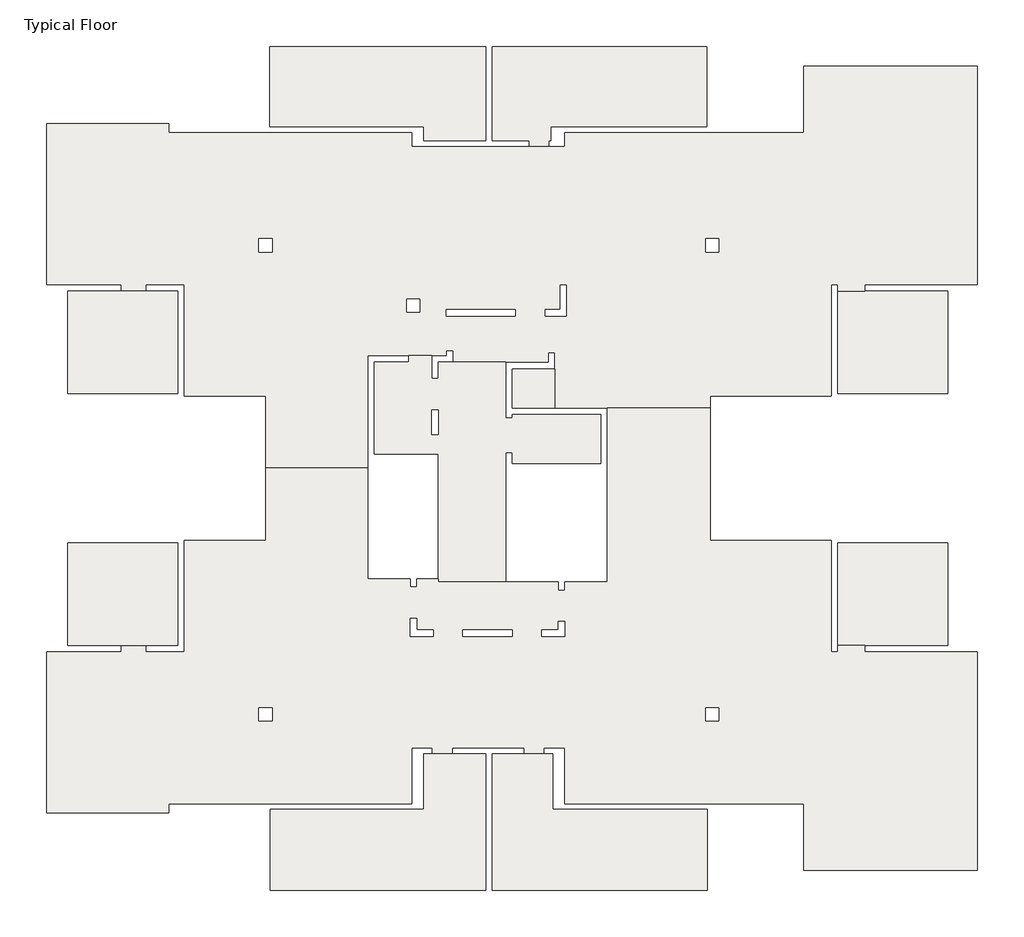
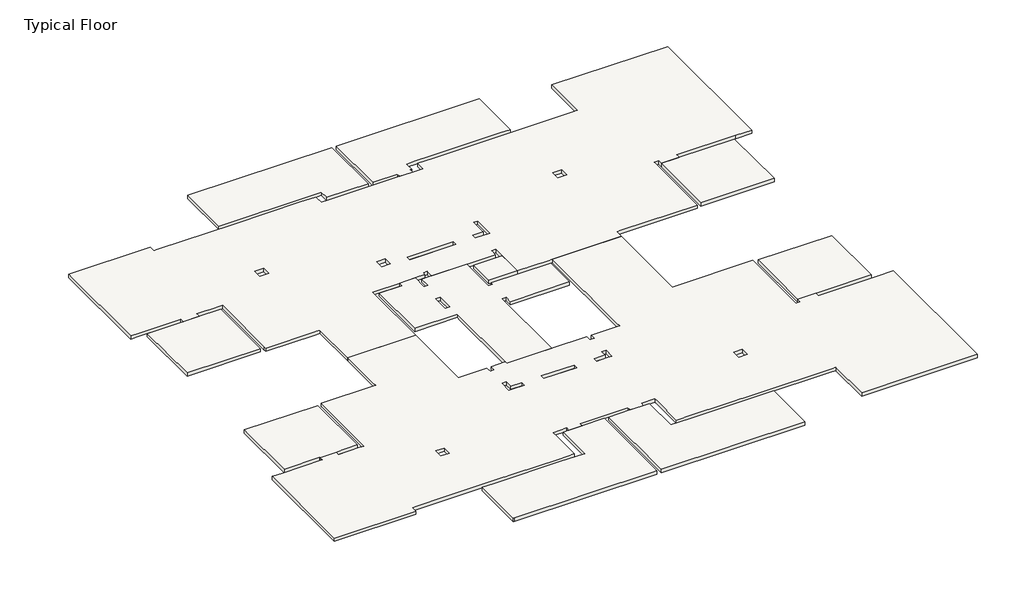
# One storey: 12 slabs.
"""IFC4 building model written with IfcOpenShell, lengths in millimetres."""

from ifc_helpers import new_model, si_unit, frame, origin, place, context, project, spatial, polyline, outline, extrude, faceted_brep, element, save

model = new_model("IFC4")

# Units and contexts
model_context = context("Model", 3, world=origin())
ifc_project = project(units=[si_unit("LENGTHUNIT", "METRE", prefix="MILLI")], contexts=[model_context])

# Site, building, storey
site = spatial("IfcSite", under=ifc_project)
building = spatial("IfcBuilding", under=site)
storey = spatial("IfcBuildingStorey", under=building, Name="Typical Floor", Elevation=3700.0)

# Slabs
placement = place(None, origin())
element("IfcSlab", 1, ObjectType="16", at=placement, inside=storey, context=model_context, shape_type="Brep", body=[
    faceted_brep([(-29879.8305532, 23917.9715458, 3540.0), (-29879.8305532, 26366.9840713, 3540.0), (-23307.4000343, 26366.9840713, 3540.0), (-23307.4000343, 23496.7461841, 3540.0), (-25199.7256887, 23496.7461841, 3540.0), (-25199.7256887, 23917.9715458, 3540.0), (-25559.7256887, 23917.9715458, 3540.0), (-26241.1471859, 23917.9715458, 3540.0), (-29280.7432632, 23917.9715458, 3540.0), (-29879.8305532, 26366.9840713, 3700.0), (-29879.8305532, 23917.9715458, 3700.0), (-29280.7432632, 23917.9715458, 3700.0), (-26241.1471859, 23917.9715458, 3700.0), (-25559.7256887, 23917.9715458, 3700.0), (-25199.7256887, 23917.9715458, 3700.0), (-25199.7256887, 23496.7461841, 3700.0), (-23307.4000343, 23496.7461841, 3700.0), (-23307.4000343, 26366.9840713, 3700.0)], [[[0, 1, 2, 3, 4, 5, 6, 7, 8]], [[9, 10, 11, 12, 13, 14, 15, 16, 17]], [[1, 0, 10, 9]], [[2, 1, 9, 17]], [[3, 2, 17, 16]], [[4, 3, 16, 15]], [[5, 4, 15, 14]], [[5, 14, 13, 12, 11, 10, 0, 8, 7, 6]]]),
])
element("IfcSlab", 2, ObjectType="16", at=placement, inside=storey, context=model_context, shape_type="Brep", body=[
    faceted_brep([(-21979.7256887, 23496.7461841, 3540.0), (-23107.4000343, 23496.7461841, 3540.0), (-23107.4000343, 26366.9840713, 3540.0), (-22980.4228437, 26366.9840713, 3540.0), (-16580.4228437, 26366.9840713, 3540.0), (-16580.4228437, 23917.8919264, 3540.0), (-17031.2403988, 23917.8919264, 3540.0), (-20181.0054246, 23917.8919264, 3540.0), (-20900.686947, 23917.8919264, 3540.0), (-21330.686947, 23917.8919264, 3540.0), (-21330.686947, 23496.7461841, 3540.0), (-21381.1801988, 23496.7461841, 3540.0), (-21381.1801988, 23316.6665647, 3540.0), (-21979.7256887, 23316.6665647, 3540.0), (-23107.4000343, 23496.7461841, 3700.0), (-21979.7256887, 23496.7461841, 3700.0), (-21979.7256887, 23316.6665647, 3700.0), (-21381.1801988, 23316.6665647, 3700.0), (-21381.1801988, 23496.7461841, 3700.0), (-21330.686947, 23496.7461841, 3700.0), (-21330.686947, 23917.8919264, 3700.0), (-20900.686947, 23917.8919264, 3700.0), (-20181.0054246, 23917.8919264, 3700.0), (-17031.2403988, 23917.8919264, 3700.0), (-16580.4228437, 23917.8919264, 3700.0), (-16580.4228437, 26366.9840713, 3700.0), (-22980.4228437, 26366.9840713, 3700.0), (-23107.4000343, 26366.9840713, 3700.0)], [[[0, 1, 2, 3, 4, 5, 6, 7, 8, 9, 10, 11, 12, 13]], [[14, 15, 16, 17, 18, 19, 20, 21, 22, 23, 24, 25, 26, 27]], [[1, 0, 15, 14]], [[2, 1, 14, 27]], [[3, 2, 27, 26]], [[4, 3, 26, 25]], [[5, 4, 25, 24]], [[5, 24, 23, 22, 21, 20, 9, 8, 7, 6]], [[10, 9, 20, 19]], [[11, 10, 19, 18]], [[12, 11, 18, 17]], [[13, 12, 17, 16]], [[0, 13, 16, 15]]]),
])
element("IfcSlab", 3, ObjectType="16", at=placement, inside=storey, context=model_context, shape_type="Brep", body=[
    faceted_brep([(-32681.2093278, 18917.1928294, 3540.0), (-32681.2093278, 15787.8356102, 3540.0), (-36030.1898114, 15787.8356102, 3540.0), (-36030.1898114, 18917.1928294, 3540.0), (-34401.0656246, 18917.1928294, 3540.0), (-33660.2169985, 18917.1928294, 3540.0), (-32681.2093278, 18917.1928294, 3700.0), (-33660.2169985, 18917.1928294, 3700.0), (-34401.0656246, 18917.1928294, 3700.0), (-36030.1898114, 18917.1928294, 3700.0), (-36030.1898114, 15787.8356102, 3700.0), (-32681.2093278, 15787.8356102, 3700.0)], [[[0, 1, 2, 3, 4, 5]], [[6, 7, 8, 9, 10, 11]], [[1, 0, 6, 11]], [[2, 1, 11, 10]], [[3, 2, 10, 9]], [[0, 5, 4, 3, 9, 8, 7, 6]]]),
])
element("IfcSlab", 4, ObjectType="16", at=placement, inside=storey, context=model_context, shape_type="SweptSolid", body=[
    extrude(outline(polyline([(-36030.9326019, 11247.0355326), (-32680.1801017, 11247.0355326), (-32680.1801017, 8117.6783134), (-33660.2169985, 8117.6783134), (-33660.2169985, 8111.6490873), (-34401.0656246, 8111.6490873), (-34401.0656246, 8116.6490873), (-36030.9326019, 8116.6490873), (-36030.9326019, 11247.0355326)])), frame((0.0, 0.0, 3540.0), z_axis=(0.0, 0.0, 1.0), x_axis=(1.0, 0.0, 0.0)), (0.0, 0.0, 1.0), 160.0),
])
element("IfcSlab", 5, ObjectType="16", at=placement, inside=storey, context=model_context, shape_type="Brep", body=[
    faceted_brep([(-9229.8888113, 11247.0355326, 3540.0), (-9229.8888113, 8116.6490873, 3540.0), (-11760.7316116, 8116.6490873, 3540.0), (-12579.898521, 8116.6490873, 3540.0), (-12579.898521, 11247.0355326, 3540.0), (-9229.8888113, 11247.0355326, 3700.0), (-12579.898521, 11247.0355326, 3700.0), (-12579.898521, 8116.6490873, 3700.0), (-11760.7316116, 8116.6490873, 3700.0), (-9229.8888113, 8116.6490873, 3700.0)], [[[0, 1, 2, 3, 4]], [[5, 6, 7, 8, 9]], [[1, 0, 5, 9]], [[3, 2, 1, 9, 8, 7]], [[4, 3, 7, 6]], [[0, 4, 6, 5]]]),
])
element("IfcSlab", 6, ObjectType="16", at=placement, inside=storey, context=model_context, shape_type="Brep", body=[
    faceted_brep([(-12579.898521, 18918.1424361, 3540.0), (-11760.7316116, 18918.1424361, 3540.0), (-9229.8888113, 18918.1424361, 3540.0), (-9229.8888113, 15787.7559909, 3540.0), (-12579.898521, 15787.7559909, 3540.0), (-12579.898521, 18918.1424361, 3700.0), (-12579.898521, 15787.7559909, 3700.0), (-9229.8888113, 15787.7559909, 3700.0), (-9229.8888113, 18918.1424361, 3700.0), (-11760.7316116, 18918.1424361, 3700.0)], [[[0, 1, 2, 3, 4]], [[5, 6, 7, 8, 9]], [[2, 1, 0, 5, 9, 8]], [[3, 2, 8, 7]], [[4, 3, 7, 6]], [[0, 4, 6, 5]]]),
])
element("IfcSlab", 7, ObjectType="16", at=placement, inside=storey, context=model_context, shape_type="Brep", body=[
    faceted_brep([(-36680.6830632, 19117.1928294, 3540.0), (-36680.6830632, 24017.2976939, 3540.0), (-32961.782199, 24017.2976939, 3540.0), (-32961.782199, 23737.8919264, 3540.0), (-32781.782199, 23737.8919264, 3540.0), (-29280.7432632, 23737.8919264, 3540.0), (-26241.1471859, 23737.8919264, 3540.0), (-25559.7256887, 23737.8919264, 3540.0), (-25559.7256887, 23316.7461841, 3540.0), (-25199.7256887, 23316.7461841, 3540.0), (-21979.7256887, 23316.7461841, 3540.0), (-21381.1801988, 23316.7461841, 3540.0), (-20900.686947, 23316.7461841, 3540.0), (-20900.686947, 23496.7461841, 3540.0), (-20900.686947, 23737.8919264, 3540.0), (-20181.0054246, 23737.8919264, 3540.0), (-17031.2403988, 23737.8919264, 3540.0), (-13801.2403988, 23737.8919264, 3540.0), (-13621.2403988, 23737.8919264, 3540.0), (-13621.2403988, 25767.8171618, 3540.0), (-8329.623737, 25767.8171618, 3540.0), (-8329.623737, 19117.1928294, 3540.0), (-9054.8888113, 19117.1928294, 3540.0), (-9054.8888113, 19118.1424361, 3540.0), (-11760.7316116, 19118.1424361, 3540.0), (-11760.7316116, 18918.1424361, 3540.0), (-12579.898521, 18918.1424361, 3540.0), (-12579.898521, 19117.11321, 3540.0), (-12779.898521, 19117.11321, 3540.0), (-12779.898521, 15787.7559909, 3540.0), (-12779.898521, 15717.7559909, 3540.0), (-16279.8286113, 15717.7559909, 3540.0), (-16459.8286113, 15717.7559909, 3540.0), (-16459.8286113, 15347.3316778, 3540.0), (-19601.0267859, 15347.3316778, 3540.0), (-19801.0267859, 15347.3316778, 3540.0), (-21201.2598182, 15347.3316778, 3540.0), (-21201.2598182, 16546.4772259, 3540.0), (-21201.2598182, 17047.0500971, 3540.0), (-21401.2598182, 17047.0500971, 3540.0), (-21401.2598182, 16746.4772259, 3540.0), (-22500.9199794, 16746.4772259, 3540.0), (-22700.9199794, 16746.4772259, 3540.0), (-24300.1237856, 16746.4772259, 3540.0), (-24300.1237856, 17097.8511457, 3540.0), (-24500.1237856, 17097.8511457, 3540.0), (-24500.1237856, 16946.4772259, 3540.0), (-24749.9538662, 16946.4772259, 3540.0), (-24949.9538662, 16946.4772259, 3540.0), (-25650.5849954, 16946.4772259, 3540.0), (-25650.5849954, 16947.5647102, 3540.0), (-26901.5608183, 16947.5647102, 3540.0), (-26901.5608183, 16747.5647102, 3540.0), (-26901.5608183, 13517.3957617, 3540.0), (-30000.4247857, 13517.3957617, 3540.0), (-30000.4247857, 15717.7559909, 3540.0), (-30180.4247857, 15717.7559909, 3540.0), (-32481.2093278, 15717.7559909, 3540.0), (-32481.2093278, 15817.1928294, 3540.0), (-32481.2093278, 19117.1928294, 3540.0), (-32681.2093278, 19117.1928294, 3540.0), (-33660.2169985, 19117.1928294, 3540.0), (-33660.2169985, 18917.1928294, 3540.0), (-34401.0656246, 18917.1928294, 3540.0), (-34401.0656246, 19117.1928294, 3540.0), (-36030.1898114, 19117.1928294, 3540.0), (-36380.1898114, 19117.1928294, 3540.0), (-29812.3773034, 20509.605542, 3540.0), (-30212.3773034, 20509.605542, 3540.0), (-30212.3773034, 20109.605542, 3540.0), (-29812.3773034, 20109.605542, 3540.0), (-25309.8528855, 18668.3919749, 3540.0), (-25709.8528855, 18668.3919749, 3540.0), (-25709.8528855, 18268.3919749, 3540.0), (-25309.8528855, 18268.3919749, 3540.0), (-22401.4345924, 18346.7102583, 3540.0), (-24501.2112698, 18346.7102583, 3540.0), (-24501.2112698, 18146.7102583, 3540.0), (-22401.4345924, 18146.7102583, 3540.0), (-21029.8858984, 18347.7394844, 3540.0), (-21499.715979, 18347.7394844, 3540.0), (-21499.715979, 18147.7394844, 3540.0), (-20849.8858984, 18147.7394844, 3540.0), (-20849.8858984, 18347.7394844, 3540.0), (-20849.8858984, 19098.1424361, 3540.0), (-21029.8858984, 19098.1424361, 3540.0), (-16205.9170786, 20509.605542, 3540.0), (-16605.9170786, 20509.605542, 3540.0), (-16605.9170786, 20109.605542, 3540.0), (-16205.9170786, 20109.605542, 3540.0), (-36680.6830632, 24017.2976939, 3700.0), (-36680.6830632, 19117.1928294, 3700.0), (-36380.1898114, 19117.1928294, 3700.0), (-36030.1898114, 19117.1928294, 3700.0), (-34401.0656246, 19117.1928294, 3700.0), (-34401.0656246, 18917.1928294, 3700.0), (-33660.2169985, 18917.1928294, 3700.0), (-33660.2169985, 19117.1928294, 3700.0), (-32681.2093278, 19117.1928294, 3700.0), (-32481.2093278, 19117.1928294, 3700.0), (-32481.2093278, 15817.1928294, 3700.0), (-32481.2093278, 15717.7559909, 3700.0), (-30180.4247857, 15717.7559909, 3700.0), (-30000.4247857, 15717.7559909, 3700.0), (-30000.4247857, 13517.3957617, 3700.0), (-26901.5608183, 13517.3957617, 3700.0), (-26901.5608183, 16747.5647102, 3700.0), (-26901.5608183, 16947.5647102, 3700.0), (-25650.5849954, 16947.5647102, 3700.0), (-25650.5849954, 16946.4772259, 3700.0), (-24949.9538662, 16946.4772259, 3700.0), (-24749.9538662, 16946.4772259, 3700.0), (-24500.1237856, 16946.4772259, 3700.0), (-24500.1237856, 17097.8511457, 3700.0), (-24300.1237856, 17097.8511457, 3700.0), (-24300.1237856, 16746.4772259, 3700.0), (-22700.9199794, 16746.4772259, 3700.0), (-22500.9199794, 16746.4772259, 3700.0), (-21401.2598182, 16746.4772259, 3700.0), (-21401.2598182, 17047.0500971, 3700.0), (-21201.2598182, 17047.0500971, 3700.0), (-21201.2598182, 16546.4772259, 3700.0), (-21201.2598182, 15347.3316778, 3700.0), (-19801.0267859, 15347.3316778, 3700.0), (-19601.0267859, 15347.3316778, 3700.0), (-16459.8286113, 15347.3316778, 3700.0), (-16459.8286113, 15717.7559909, 3700.0), (-16279.8286113, 15717.7559909, 3700.0), (-12779.898521, 15717.7559909, 3700.0), (-12779.898521, 15787.7559909, 3700.0), (-12779.898521, 19117.11321, 3700.0), (-12579.898521, 19117.11321, 3700.0), (-12579.898521, 18918.1424361, 3700.0), (-11760.7316116, 18918.1424361, 3700.0), (-11760.7316116, 19118.1424361, 3700.0), (-9054.8888113, 19118.1424361, 3700.0), (-9054.8888113, 19117.1928294, 3700.0), (-8329.623737, 19117.1928294, 3700.0), (-8329.623737, 25767.8171618, 3700.0), (-13621.2403988, 25767.8171618, 3700.0), (-13621.2403988, 23737.8919264, 3700.0), (-13801.2403988, 23737.8919264, 3700.0), (-17031.2403988, 23737.8919264, 3700.0), (-20181.0054246, 23737.8919264, 3700.0), (-20900.686947, 23737.8919264, 3700.0), (-20900.686947, 23496.7461841, 3700.0), (-20900.686947, 23316.7461841, 3700.0), (-21381.1801988, 23316.7461841, 3700.0), (-21979.7256887, 23316.7461841, 3700.0), (-25199.7256887, 23316.7461841, 3700.0), (-25559.7256887, 23316.7461841, 3700.0), (-25559.7256887, 23737.8919264, 3700.0), (-26241.1471859, 23737.8919264, 3700.0), (-29280.7432632, 23737.8919264, 3700.0), (-32781.782199, 23737.8919264, 3700.0), (-32961.782199, 23737.8919264, 3700.0), (-32961.782199, 24017.2976939, 3700.0), (-16605.9170786, 20509.605542, 3700.0), (-16205.9170786, 20509.605542, 3700.0), (-16205.9170786, 20109.605542, 3700.0), (-16605.9170786, 20109.605542, 3700.0), (-30212.3773034, 20509.605542, 3700.0), (-29812.3773034, 20509.605542, 3700.0), (-29812.3773034, 20109.605542, 3700.0), (-30212.3773034, 20109.605542, 3700.0), (-25709.8528855, 18668.3919749, 3700.0), (-25309.8528855, 18668.3919749, 3700.0), (-25309.8528855, 18268.3919749, 3700.0), (-25709.8528855, 18268.3919749, 3700.0), (-21499.715979, 18347.7394844, 3700.0), (-21029.8858984, 18347.7394844, 3700.0), (-21029.8858984, 19098.1424361, 3700.0), (-20849.8858984, 19098.1424361, 3700.0), (-20849.8858984, 18347.7394844, 3700.0), (-20849.8858984, 18147.7394844, 3700.0), (-21499.715979, 18147.7394844, 3700.0), (-24501.2112698, 18346.7102583, 3700.0), (-22401.4345924, 18346.7102583, 3700.0), (-22401.4345924, 18146.7102583, 3700.0), (-24501.2112698, 18146.7102583, 3700.0)], [[[0, 1, 2, 3, 4, 5, 6, 7, 8, 9, 10, 11, 12, 13, 14, 15, 16, 17, 18, 19, 20, 21, 22, 23, 24, 25, 26, 27, 28, 29, 30, 31, 32, 33, 34, 35, 36, 37, 38, 39, 40, 41, 42, 43, 44, 45, 46, 47, 48, 49, 50, 51, 52, 53, 54, 55, 56, 57, 58, 59, 60, 61, 62, 63, 64, 65, 66], [67, 68, 69, 70], [71, 72, 73, 74], [75, 76, 77, 78], [79, 80, 81, 82, 83, 84, 85], [86, 87, 88, 89]], [[90, 91, 92, 93, 94, 95, 96, 97, 98, 99, 100, 101, 102, 103, 104, 105, 106, 107, 108, 109, 110, 111, 112, 113, 114, 115, 116, 117, 118, 119, 120, 121, 122, 123, 124, 125, 126, 127, 128, 129, 130, 131, 132, 133, 134, 135, 136, 137, 138, 139, 140, 141, 142, 143, 144, 145, 146, 147, 148, 149, 150, 151, 152, 153, 154, 155, 156], [157, 158, 159, 160], [161, 162, 163, 164], [165, 166, 167, 168], [169, 170, 171, 172, 173, 174, 175], [176, 177, 178, 179]], [[1, 0, 91, 90]], [[2, 1, 90, 156]], [[3, 2, 156, 155]], [[3, 155, 154, 153, 152, 151, 7, 6, 5, 4]], [[8, 7, 151, 150]], [[8, 150, 149, 148, 147, 146, 12, 11, 10, 9]], [[12, 146, 145, 144, 14, 13]], [[14, 144, 143, 142, 141, 140, 18, 17, 16, 15]], [[19, 18, 140, 139]], [[20, 19, 139, 138]], [[21, 20, 138, 137]], [[21, 137, 136, 22]], [[133, 25, 24, 134]], [[26, 25, 133, 132]], [[27, 26, 132, 131]], [[28, 27, 131, 130]], [[28, 130, 129, 128, 30, 29]], [[30, 128, 127, 126, 32, 31]], [[33, 32, 126, 125]], [[33, 125, 124, 123, 122, 36, 35, 34]], [[37, 36, 122, 121]], [[38, 37, 121, 120]], [[39, 38, 120, 119]], [[40, 39, 119, 118]], [[40, 118, 117, 116, 42, 41]], [[43, 42, 116, 115]], [[44, 43, 115, 114]], [[45, 44, 114, 113]], [[46, 45, 113, 112]], [[46, 112, 111, 110, 48, 47]], [[49, 48, 110, 109]], [[105, 53, 52, 51, 107, 106]], [[54, 53, 105, 104]], [[55, 54, 104, 103]], [[55, 103, 102, 101, 57, 56]], [[58, 57, 101, 100]], [[59, 58, 100, 99]], [[59, 99, 98, 97, 61, 60]], [[62, 61, 97, 96]], [[63, 62, 96, 95]], [[64, 63, 95, 94]], [[64, 94, 93, 92, 91, 0, 66, 65]], [[68, 67, 162, 161]], [[69, 68, 161, 164]], [[70, 69, 164, 163]], [[67, 70, 163, 162]], [[72, 71, 166, 165]], [[73, 72, 165, 168]], [[74, 73, 168, 167]], [[71, 74, 167, 166]], [[76, 75, 177, 176]], [[77, 76, 176, 179]], [[78, 77, 179, 178]], [[75, 78, 178, 177]], [[80, 79, 170, 169]], [[81, 80, 169, 175]], [[82, 81, 175, 174]], [[82, 174, 173, 172, 84, 83]], [[85, 84, 172, 171]], [[79, 85, 171, 170]], [[87, 86, 158, 157]], [[88, 87, 157, 160]], [[89, 88, 160, 159]], [[86, 89, 159, 158]], [[23, 135, 134, 24]], [[135, 23, 22, 136]], [[50, 108, 107, 51]], [[108, 50, 49, 109]]]),
])
element("IfcSlab", 8, ObjectType="16", at=placement, inside=storey, context=model_context, shape_type="Brep", body=[
    faceted_brep([(-30000.4247857, 13517.3957617, 3540.0), (-26901.5608183, 13517.3957617, 3540.0), (-26901.5608183, 10146.5743227, 3540.0), (-26701.5608183, 10146.5743227, 3540.0), (-25599.7839467, 10146.5743227, 3540.0), (-25599.7839467, 9896.8025002, 3540.0), (-25399.7839467, 9896.8025002, 3540.0), (-25399.7839467, 10146.5743227, 3540.0), (-24750.9830923, 10146.5743227, 3540.0), (-24750.9830923, 10047.0889358, 3540.0), (-22699.8907532, 10047.0889358, 3540.0), (-21100.686947, 10047.0889358, 3540.0), (-21100.686947, 9797.3171133, 3540.0), (-20900.686947, 9797.3171133, 3540.0), (-20900.686947, 10047.0889358, 3540.0), (-19601.0267859, 10047.0889358, 3540.0), (-19601.0267859, 10247.0889358, 3540.0), (-19601.0267859, 15347.3316778, 3540.0), (-16459.8286113, 15347.3316778, 3540.0), (-16459.8286113, 11497.0355326, 3540.0), (-16459.8286113, 11317.0355326, 3540.0), (-12779.898521, 11317.0355326, 3540.0), (-12779.898521, 11247.0355326, 3540.0), (-12779.898521, 7917.6783134, 3540.0), (-12579.898521, 7917.6783134, 3540.0), (-12579.898521, 8116.6490873, 3540.0), (-11760.7316116, 8116.6490873, 3540.0), (-11760.7316116, 7916.6490873, 3540.0), (-9054.8888113, 7916.6490873, 3540.0), (-9054.8888113, 7917.598694, 3540.0), (-8329.623737, 7917.598694, 3540.0), (-8329.623737, 1267.053981, 3540.0), (-13621.2403988, 1267.053981, 3540.0), (-13621.2403988, 3296.899597, 3540.0), (-13801.2403988, 3296.899597, 3540.0), (-17179.5101337, 3296.899597, 3540.0), (-20181.0054246, 3296.899597, 3540.0), (-20900.5277083, 3296.899597, 3540.0), (-20900.5277083, 4816.6180163, 3540.0), (-20900.5277083, 4996.6180163, 3540.0), (-21531.4666344, 4996.6180163, 3540.0), (-21531.4666344, 4816.6180163, 3540.0), (-22130.4956663, 4816.6180163, 3540.0), (-22130.4956663, 4996.6180163, 3540.0), (-24329.7577306, 4996.6180163, 3540.0), (-24329.7577306, 4816.6180163, 3540.0), (-24930.9034729, 4816.6180163, 3540.0), (-24930.9034729, 4996.6180163, 3540.0), (-25559.7256887, 4996.6180163, 3540.0), (-25559.7256887, 4816.6180163, 3540.0), (-25559.7256887, 3296.899597, 3540.0), (-26281.3646827, 3296.899597, 3540.0), (-29280.7432632, 3296.899597, 3540.0), (-32781.782199, 3296.899597, 3540.0), (-32961.782199, 3296.899597, 3540.0), (-32961.782199, 3017.5734489, 3540.0), (-36680.6830632, 3017.5734489, 3540.0), (-36680.6830632, 7917.598694, 3540.0), (-36661.0656246, 7917.598694, 3540.0), (-36205.9326019, 7917.598694, 3540.0), (-36205.9326019, 7916.6490873, 3540.0), (-34401.0656246, 7916.6490873, 3540.0), (-34401.0656246, 8111.6490873, 3540.0), (-33660.2169985, 8111.6490873, 3540.0), (-33660.2169985, 7917.6783134, 3540.0), (-32680.1801017, 7917.6783134, 3540.0), (-32480.1801017, 7917.6783134, 3540.0), (-32480.1801017, 11247.0355326, 3540.0), (-32480.1801017, 11317.0355326, 3540.0), (-30000.4247857, 11317.0355326, 3540.0), (-30000.4247857, 11497.0355326, 3540.0), (-22500.9199794, 8596.0548548, 3540.0), (-24001.6676248, 8596.0548548, 3540.0), (-24001.6676248, 8396.0548548, 3540.0), (-22500.9199794, 8396.0548548, 3540.0), (-29812.3773034, 6215.7849257, 3540.0), (-30212.3773034, 6215.7849257, 3540.0), (-30212.3773034, 5815.7849257, 3540.0), (-29812.3773034, 5815.7849257, 3540.0), (-16205.9170786, 6215.8431838, 3540.0), (-16605.9170786, 6215.8431838, 3540.0), (-16605.9170786, 5815.8431838, 3540.0), (-16205.9170786, 5815.8431838, 3540.0), (-21601.3180763, 8596.0548548, 3540.0), (-21601.3180763, 8396.0548548, 3540.0), (-21100.686947, 8396.0548548, 3540.0), (-20900.686947, 8396.0548548, 3540.0), (-20900.686947, 8846.9141616, 3540.0), (-21100.686947, 8846.9141616, 3540.0), (-21100.686947, 8596.0548548, 3540.0), (-24901.2695279, 8596.0548548, 3540.0), (-25399.7839467, 8596.0548548, 3540.0), (-25399.7839467, 8946.3995485, 3540.0), (-25599.7839467, 8946.3995485, 3540.0), (-25599.7839467, 8396.0548548, 3540.0), (-25399.7839467, 8396.0548548, 3540.0), (-24901.2695279, 8396.0548548, 3540.0), (-26901.5608183, 13517.3957617, 3700.0), (-30000.4247857, 13517.3957617, 3700.0), (-30000.4247857, 11497.0355326, 3700.0), (-30000.4247857, 11317.0355326, 3700.0), (-32480.1801017, 11317.0355326, 3700.0), (-32480.1801017, 11247.0355326, 3700.0), (-32480.1801017, 7917.6783134, 3700.0), (-32680.1801017, 7917.6783134, 3700.0), (-33660.2169985, 7917.6783134, 3700.0), (-33660.2169985, 8111.6490873, 3700.0), (-34401.0656246, 8111.6490873, 3700.0), (-34401.0656246, 7916.6490873, 3700.0), (-36205.9326019, 7916.6490873, 3700.0), (-36205.9326019, 7917.598694, 3700.0), (-36661.0656246, 7917.598694, 3700.0), (-36680.6830632, 7917.598694, 3700.0), (-36680.6830632, 3017.5734489, 3700.0), (-32961.782199, 3017.5734489, 3700.0), (-32961.782199, 3296.899597, 3700.0), (-32781.782199, 3296.899597, 3700.0), (-29280.7432632, 3296.899597, 3700.0), (-26281.3646827, 3296.899597, 3700.0), (-25559.7256887, 3296.899597, 3700.0), (-25559.7256887, 4816.6180163, 3700.0), (-25559.7256887, 4996.6180163, 3700.0), (-24930.9034729, 4996.6180163, 3700.0), (-24930.9034729, 4816.6180163, 3700.0), (-24329.7577306, 4816.6180163, 3700.0), (-24329.7577306, 4996.6180163, 3700.0), (-22130.4956663, 4996.6180163, 3700.0), (-22130.4956663, 4816.6180163, 3700.0), (-21531.4666344, 4816.6180163, 3700.0), (-21531.4666344, 4996.6180163, 3700.0), (-20900.5277083, 4996.6180163, 3700.0), (-20900.5277083, 4816.6180163, 3700.0), (-20900.5277083, 3296.899597, 3700.0), (-20181.0054246, 3296.899597, 3700.0), (-17179.5101337, 3296.899597, 3700.0), (-13801.2403988, 3296.899597, 3700.0), (-13621.2403988, 3296.899597, 3700.0), (-13621.2403988, 1267.053981, 3700.0), (-8329.623737, 1267.053981, 3700.0), (-8329.623737, 7917.598694, 3700.0), (-9054.8888113, 7917.598694, 3700.0), (-9054.8888113, 7916.6490873, 3700.0), (-11760.7316116, 7916.6490873, 3700.0), (-11760.7316116, 8116.6490873, 3700.0), (-12579.898521, 8116.6490873, 3700.0), (-12579.898521, 7917.6783134, 3700.0), (-12779.898521, 7917.6783134, 3700.0), (-12779.898521, 11247.0355326, 3700.0), (-12779.898521, 11317.0355326, 3700.0), (-16459.8286113, 11317.0355326, 3700.0), (-16459.8286113, 11497.0355326, 3700.0), (-16459.8286113, 15347.3316778, 3700.0), (-19601.0267859, 15347.3316778, 3700.0), (-19601.0267859, 10247.0889358, 3700.0), (-19601.0267859, 10047.0889358, 3700.0), (-20900.686947, 10047.0889358, 3700.0), (-20900.686947, 9797.3171133, 3700.0), (-21100.686947, 9797.3171133, 3700.0), (-21100.686947, 10047.0889358, 3700.0), (-22699.8907532, 10047.0889358, 3700.0), (-24750.9830923, 10047.0889358, 3700.0), (-24750.9830923, 10146.5743227, 3700.0), (-25399.7839467, 10146.5743227, 3700.0), (-25399.7839467, 9896.8025002, 3700.0), (-25599.7839467, 9896.8025002, 3700.0), (-25599.7839467, 10146.5743227, 3700.0), (-26701.5608183, 10146.5743227, 3700.0), (-26901.5608183, 10146.5743227, 3700.0), (-30212.3773034, 6215.7849257, 3700.0), (-29812.3773034, 6215.7849257, 3700.0), (-29812.3773034, 5815.7849257, 3700.0), (-30212.3773034, 5815.7849257, 3700.0), (-16605.9170786, 6215.8431838, 3700.0), (-16205.9170786, 6215.8431838, 3700.0), (-16205.9170786, 5815.8431838, 3700.0), (-16605.9170786, 5815.8431838, 3700.0), (-25399.7839467, 8596.0548548, 3700.0), (-24901.2695279, 8596.0548548, 3700.0), (-24901.2695279, 8396.0548548, 3700.0), (-25399.7839467, 8396.0548548, 3700.0), (-25599.7839467, 8396.0548548, 3700.0), (-25599.7839467, 8946.3995485, 3700.0), (-25399.7839467, 8946.3995485, 3700.0), (-24001.6676248, 8596.0548548, 3700.0), (-22500.9199794, 8596.0548548, 3700.0), (-22500.9199794, 8396.0548548, 3700.0), (-24001.6676248, 8396.0548548, 3700.0), (-21601.3180763, 8396.0548548, 3700.0), (-21601.3180763, 8596.0548548, 3700.0), (-21100.686947, 8596.0548548, 3700.0), (-21100.686947, 8846.9141616, 3700.0), (-20900.686947, 8846.9141616, 3700.0), (-20900.686947, 8396.0548548, 3700.0), (-21100.686947, 8396.0548548, 3700.0)], [[[0, 1, 2, 3, 4, 5, 6, 7, 8, 9, 10, 11, 12, 13, 14, 15, 16, 17, 18, 19, 20, 21, 22, 23, 24, 25, 26, 27, 28, 29, 30, 31, 32, 33, 34, 35, 36, 37, 38, 39, 40, 41, 42, 43, 44, 45, 46, 47, 48, 49, 50, 51, 52, 53, 54, 55, 56, 57, 58, 59, 60, 61, 62, 63, 64, 65, 66, 67, 68, 69, 70], [71, 72, 73, 74], [75, 76, 77, 78], [79, 80, 81, 82], [83, 84, 85, 86, 87, 88, 89], [90, 91, 92, 93, 94, 95, 96]], [[97, 98, 99, 100, 101, 102, 103, 104, 105, 106, 107, 108, 109, 110, 111, 112, 113, 114, 115, 116, 117, 118, 119, 120, 121, 122, 123, 124, 125, 126, 127, 128, 129, 130, 131, 132, 133, 134, 135, 136, 137, 138, 139, 140, 141, 142, 143, 144, 145, 146, 147, 148, 149, 150, 151, 152, 153, 154, 155, 156, 157, 158, 159, 160, 161, 162, 163, 164, 165, 166, 167], [168, 169, 170, 171], [172, 173, 174, 175], [176, 177, 178, 179, 180, 181, 182], [183, 184, 185, 186], [187, 188, 189, 190, 191, 192, 193]], [[1, 0, 98, 97]], [[2, 1, 97, 167]], [[2, 167, 166, 165, 4, 3]], [[5, 4, 165, 164]], [[6, 5, 164, 163]], [[7, 6, 163, 162]], [[8, 7, 162, 161]], [[9, 8, 161, 160]], [[9, 160, 159, 158, 11, 10]], [[12, 11, 158, 157]], [[13, 12, 157, 156]], [[14, 13, 156, 155]], [[15, 14, 155, 154]], [[15, 154, 153, 152, 17, 16]], [[18, 17, 152, 151]], [[18, 151, 150, 149, 20, 19]], [[21, 20, 149, 148]], [[21, 148, 147, 146, 23, 22]], [[24, 23, 146, 145]], [[25, 24, 145, 144]], [[26, 25, 144, 143]], [[26, 143, 142, 27]], [[139, 30, 29, 140]], [[31, 30, 139, 138]], [[32, 31, 138, 137]], [[33, 32, 137, 136]], [[33, 136, 135, 134, 133, 132, 37, 36, 35, 34]], [[37, 132, 131, 130, 39, 38]], [[40, 39, 130, 129]], [[41, 40, 129, 128]], [[42, 41, 128, 127]], [[43, 42, 127, 126]], [[44, 43, 126, 125]], [[45, 44, 125, 124]], [[46, 45, 124, 123]], [[47, 46, 123, 122]], [[48, 47, 122, 121]], [[48, 121, 120, 119, 50, 49]], [[50, 119, 118, 117, 116, 115, 54, 53, 52, 51]], [[55, 54, 115, 114]], [[56, 55, 114, 113]], [[57, 56, 113, 112]], [[58, 57, 112, 111]], [[58, 111, 110, 59]], [[107, 62, 61, 108]], [[105, 64, 63, 106]], [[64, 105, 104, 103, 66, 65]], [[66, 103, 102, 101, 68, 67]], [[69, 68, 101, 100]], [[69, 100, 99, 98, 0, 70]], [[72, 71, 184, 183]], [[73, 72, 183, 186]], [[74, 73, 186, 185]], [[71, 74, 185, 184]], [[76, 75, 169, 168]], [[77, 76, 168, 171]], [[78, 77, 171, 170]], [[75, 78, 170, 169]], [[80, 79, 173, 172]], [[81, 80, 172, 175]], [[82, 81, 175, 174]], [[79, 82, 174, 173]], [[84, 83, 188, 187]], [[84, 187, 193, 192, 86, 85]], [[87, 86, 192, 191]], [[88, 87, 191, 190]], [[89, 88, 190, 189]], [[83, 89, 189, 188]], [[91, 90, 177, 176]], [[92, 91, 176, 182]], [[93, 92, 182, 181]], [[94, 93, 181, 180]], [[94, 180, 179, 178, 96, 95]], [[90, 96, 178, 177]], [[63, 62, 107, 106]], [[60, 109, 108, 61]], [[109, 60, 59, 110]], [[27, 142, 141, 28]], [[28, 141, 140, 29]]]),
])
element("IfcSlab", 9, ObjectType="16", at=placement, inside=storey, context=model_context, shape_type="Brep", body=[
    faceted_brep([(-25650.5849954, 16946.4772259, 3540.0), (-24949.9538662, 16946.4772259, 3540.0), (-24949.9538662, 16246.9335809, 3540.0), (-24749.9538662, 16246.9335809, 3540.0), (-24749.9538662, 16746.4772259, 3540.0), (-24500.1237856, 16746.4772259, 3540.0), (-24300.1237856, 16746.4772259, 3540.0), (-22700.9199794, 16746.4772259, 3540.0), (-22700.9199794, 15046.7588067, 3540.0), (-22500.9199794, 15046.7588067, 3540.0), (-22500.9199794, 15147.3316778, 3540.0), (-19801.0267859, 15147.3316778, 3540.0), (-19801.0267859, 13656.870468, 3540.0), (-22499.8907532, 13656.870468, 3540.0), (-22499.8907532, 13996.870468, 3540.0), (-22699.8907532, 13996.870468, 3540.0), (-22699.8907532, 10247.0889358, 3540.0), (-22699.8907532, 10047.0889358, 3540.0), (-24750.9830923, 10047.0889358, 3540.0), (-24750.9830923, 10146.5743227, 3540.0), (-24750.9830923, 10346.5743227, 3540.0), (-24750.9830923, 13748.1861297, 3540.0), (-24750.9830923, 13948.1861297, 3540.0), (-26701.5608183, 13948.1861297, 3540.0), (-26701.5608183, 16747.5647102, 3540.0), (-25650.5849954, 16747.5647102, 3540.0), (-24949.9538662, 15296.5306292, 3540.0), (-24949.9538662, 14547.2151617, 3540.0), (-24749.9538662, 14547.2151617, 3540.0), (-24749.9538662, 15296.5306292, 3540.0), (-24949.9538662, 16946.4772259, 3700.0), (-25650.5849954, 16946.4772259, 3700.0), (-25650.5849954, 16747.5647102, 3700.0), (-26701.5608183, 16747.5647102, 3700.0), (-26701.5608183, 13948.1861297, 3700.0), (-24750.9830923, 13948.1861297, 3700.0), (-24750.9830923, 13748.1861297, 3700.0), (-24750.9830923, 10346.5743227, 3700.0), (-24750.9830923, 10146.5743227, 3700.0), (-24750.9830923, 10047.0889358, 3700.0), (-22699.8907532, 10047.0889358, 3700.0), (-22699.8907532, 10247.0889358, 3700.0), (-22699.8907532, 13996.870468, 3700.0), (-22499.8907532, 13996.870468, 3700.0), (-22499.8907532, 13656.870468, 3700.0), (-19801.0267859, 13656.870468, 3700.0), (-19801.0267859, 15147.3316778, 3700.0), (-22500.9199794, 15147.3316778, 3700.0), (-22500.9199794, 15046.7588067, 3700.0), (-22700.9199794, 15046.7588067, 3700.0), (-22700.9199794, 16746.4772259, 3700.0), (-24300.1237856, 16746.4772259, 3700.0), (-24500.1237856, 16746.4772259, 3700.0), (-24749.9538662, 16746.4772259, 3700.0), (-24749.9538662, 16246.9335809, 3700.0), (-24949.9538662, 16246.9335809, 3700.0), (-24949.9538662, 14547.2151617, 3700.0), (-24949.9538662, 15296.5306292, 3700.0), (-24749.9538662, 15296.5306292, 3700.0), (-24749.9538662, 14547.2151617, 3700.0)], [[[0, 1, 2, 3, 4, 5, 6, 7, 8, 9, 10, 11, 12, 13, 14, 15, 16, 17, 18, 19, 20, 21, 22, 23, 24, 25], [26, 27, 28, 29]], [[30, 31, 32, 33, 34, 35, 36, 37, 38, 39, 40, 41, 42, 43, 44, 45, 46, 47, 48, 49, 50, 51, 52, 53, 54, 55], [56, 57, 58, 59]], [[26, 57, 56, 27]], [[58, 29, 28, 59]], [[27, 56, 59, 28]], [[57, 26, 29, 58]], [[1, 0, 31, 30]], [[2, 1, 30, 55]], [[3, 2, 55, 54]], [[4, 3, 54, 53]], [[4, 53, 52, 51, 50, 7, 6, 5]], [[8, 7, 50, 49]], [[9, 8, 49, 48]], [[10, 9, 48, 47]], [[11, 10, 47, 46]], [[12, 11, 46, 45]], [[13, 12, 45, 44]], [[14, 13, 44, 43]], [[15, 14, 43, 42]], [[15, 42, 41, 40, 17, 16]], [[18, 17, 40, 39]], [[18, 39, 38, 37, 36, 35, 22, 21, 20, 19]], [[23, 22, 35, 34]], [[24, 23, 34, 33]], [[25, 24, 33, 32]], [[0, 25, 32, 31]]]),
])
element("IfcSlab", 10, ObjectType="16", at=placement, inside=storey, context=model_context, shape_type="Brep", body=[
    faceted_brep([(-21201.2598182, 16546.4772259, 3540.0), (-21201.2598182, 15347.3316778, 3540.0), (-22500.9199794, 15347.3316778, 3540.0), (-22500.9199794, 16546.4772259, 3540.0), (-21201.2598182, 15347.3316778, 3700.0), (-21201.2598182, 16546.4772259, 3700.0), (-21401.2598182, 16546.4772259, 3700.0), (-22500.9199794, 16546.4772259, 3700.0), (-22500.9199794, 15347.3316778, 3700.0)], [[[0, 1, 2, 3]], [[4, 5, 6, 7, 8]], [[1, 0, 5, 4]], [[2, 1, 4, 8]], [[3, 2, 8, 7]], [[0, 3, 7, 6, 5]]]),
])
element("IfcSlab", 11, ObjectType="16", at=placement, inside=storey, context=model_context, shape_type="Brep", body=[
    faceted_brep([(-25199.7256887, 3116.899597, 3540.0), (-25199.7256887, 4816.6180163, 3540.0), (-24930.9034729, 4816.6180163, 3540.0), (-24329.7577306, 4816.6180163, 3540.0), (-23311.6200473, 4816.6180163, 3540.0), (-23311.6200473, 659.7166846, 3540.0), (-29811.6200473, 659.7166846, 3540.0), (-29861.4923547, 659.7166846, 3540.0), (-29861.4923547, 3116.899597, 3540.0), (-29280.7432632, 3116.899597, 3540.0), (-26281.3646827, 3116.899597, 3540.0), (-25559.7256887, 3116.899597, 3540.0), (-25199.7256887, 4816.6180163, 3700.0), (-25199.7256887, 3116.899597, 3700.0), (-25559.7256887, 3116.899597, 3700.0), (-26281.3646827, 3116.899597, 3700.0), (-29280.7432632, 3116.899597, 3700.0), (-29861.4923547, 3116.899597, 3700.0), (-29861.4923547, 659.7166846, 3700.0), (-29811.6200473, 659.7166846, 3700.0), (-23311.6200473, 659.7166846, 3700.0), (-23311.6200473, 4816.6180163, 3700.0), (-24329.7577306, 4816.6180163, 3700.0), (-24930.9034729, 4816.6180163, 3700.0)], [[[0, 1, 2, 3, 4, 5, 6, 7, 8, 9, 10, 11]], [[12, 13, 14, 15, 16, 17, 18, 19, 20, 21, 22, 23]], [[13, 0, 11, 10, 9, 8, 17, 16, 15, 14]], [[1, 0, 13, 12]], [[1, 12, 23, 22, 21, 4, 3, 2]], [[5, 4, 21, 20]], [[6, 5, 20, 19]], [[7, 6, 19, 18]], [[8, 7, 18, 17]]]),
])
element("IfcSlab", 12, ObjectType="16", at=placement, inside=storey, context=model_context, shape_type="Brep", body=[
    faceted_brep([(-16561.2977307, 3116.899597, 3540.0), (-16561.2977307, 659.7166846, 3540.0), (-23111.6200473, 659.7166846, 3540.0), (-23111.6200473, 4816.6180163, 3540.0), (-22130.4956663, 4816.6180163, 3540.0), (-21531.4666344, 4816.6180163, 3540.0), (-21260.5277083, 4816.6180163, 3540.0), (-21260.5277083, 3116.899597, 3540.0), (-20900.5277083, 3116.899597, 3540.0), (-20181.0054246, 3116.899597, 3540.0), (-17179.5101337, 3116.899597, 3540.0), (-16561.2977307, 659.7166846, 3700.0), (-16561.2977307, 3116.899597, 3700.0), (-17179.5101337, 3116.899597, 3700.0), (-20181.0054246, 3116.899597, 3700.0), (-20900.5277083, 3116.899597, 3700.0), (-21260.5277083, 3116.899597, 3700.0), (-21260.5277083, 4816.6180163, 3700.0), (-21531.4666344, 4816.6180163, 3700.0), (-22130.4956663, 4816.6180163, 3700.0), (-23111.6200473, 4816.6180163, 3700.0), (-23111.6200473, 659.7166846, 3700.0)], [[[0, 1, 2, 3, 4, 5, 6, 7, 8, 9, 10]], [[11, 12, 13, 14, 15, 16, 17, 18, 19, 20, 21]], [[16, 7, 6, 17]], [[7, 16, 15, 14, 13, 12, 0, 10, 9, 8]], [[1, 0, 12, 11]], [[2, 1, 11, 21]], [[2, 21, 20, 3]], [[3, 20, 19, 18, 17, 6, 5, 4]]]),
])

save(model, "model.ifc")

# Revit data of these elements
# Type "16"
#   Function = 0
#   Layers, outside or top first: 16 cm "Concrete" (function 1)
# Element 1 (IfcSlab, "16")
#   Mark = "S1"
#   SOFiSTiK_AMG_Comments = ""
#   built-in parameter 1001955 = -1.5708 (stored number, unit not read)
#   Height Offset From Level = 0 cm
#   built-in parameter 1001954 = 1
#   SOFiSTiK_AMG_Scheduled = yes
#   SOFiSTiK_AMG_Adjusted = yes
#   Phase Created = New Construction
#   Materials on its faces: "Concrete"
# Element 2 (IfcSlab, "16")
#   Mark = "S2"
#   SOFiSTiK_AMG_Comments = ""
#   Height Offset From Level = 0 cm
#   built-in parameter 1001954 = 1
#   SOFiSTiK_AMG_Scheduled = yes
#   SOFiSTiK_AMG_Adjusted = yes
#   Phase Created = New Construction
#   Materials on its faces: "Concrete"
# Element 3 (IfcSlab, "16")
#   Mark = "S3"
#   SOFiSTiK_AMG_Comments = ""
#   Height Offset From Level = 0 cm
#   built-in parameter 1001954 = 1
#   SOFiSTiK_AMG_Scheduled = yes
#   SOFiSTiK_AMG_Adjusted = yes
#   Phase Created = New Construction
#   Materials on its faces: "Concrete"
# Element 4 (IfcSlab, "16")
#   Mark = "S4"
#   SOFiSTiK_AMG_Comments = ""
#   Height Offset From Level = 0 cm
#   built-in parameter 1001954 = 1
#   SOFiSTiK_AMG_Scheduled = yes
#   SOFiSTiK_AMG_Adjusted = yes
#   Phase Created = New Construction
#   Materials on its faces: "Concrete"
# Element 5 (IfcSlab, "16")
#   Mark = "S5"
#   SOFiSTiK_AMG_Comments = ""
#   Height Offset From Level = 0 cm
#   built-in parameter 1001954 = 1
#   SOFiSTiK_AMG_Scheduled = yes
#   SOFiSTiK_AMG_Adjusted = yes
#   Phase Created = New Construction
#   Materials on its faces: "Concrete"
# Element 6 (IfcSlab, "16")
#   Mark = "S6"
#   SOFiSTiK_AMG_Comments = ""
#   built-in parameter 1001955 = 3.14159 (stored number, unit not read)
#   Height Offset From Level = 0 cm
#   built-in parameter 1001954 = 1
#   SOFiSTiK_AMG_Scheduled = yes
#   SOFiSTiK_AMG_Adjusted = yes
#   Phase Created = New Construction
#   Materials on its faces: "Concrete"
# Element 7 (IfcSlab, "16")
#   Mark = "S7"
#   SOFiSTiK_AMG_Comments = ""
#   built-in parameter 1001955 = -1.5708 (stored number, unit not read)
#   Height Offset From Level = 0 cm
#   built-in parameter 1001954 = 1
#   SOFiSTiK_AMG_Scheduled = yes
#   SOFiSTiK_AMG_Adjusted = yes
#   Phase Created = New Construction
#   Materials on its faces: "Concrete"
# Element 8 (IfcSlab, "16")
#   Mark = "S8"
#   SOFiSTiK_AMG_Comments = ""
#   built-in parameter 1001955 = 3.14159 (stored number, unit not read)
#   Height Offset From Level = 0 cm
#   built-in parameter 1001954 = 1
#   SOFiSTiK_AMG_Scheduled = yes
#   SOFiSTiK_AMG_Adjusted = yes
#   Phase Created = New Construction
#   Materials on its faces: "Concrete"
# Element 9 (IfcSlab, "16")
#   Mark = "S9"
#   SOFiSTiK_AMG_Comments = ""
#   built-in parameter 1001955 = 1.5708 (stored number, unit not read)
#   Height Offset From Level = 0 cm
#   built-in parameter 1001954 = 1
#   SOFiSTiK_AMG_Scheduled = yes
#   SOFiSTiK_AMG_Adjusted = yes
#   Phase Created = New Construction
#   Materials on its faces: "Concrete"
# Element 10 (IfcSlab, "16")
#   Mark = "S10"
#   SOFiSTiK_AMG_Comments = ""
#   Height Offset From Level = 0 cm
#   built-in parameter 1001954 = 1
#   SOFiSTiK_AMG_Scheduled = yes
#   SOFiSTiK_AMG_Adjusted = yes
#   Phase Created = New Construction
#   Materials on its faces: "Concrete"
# Element 11 (IfcSlab, "16")
#   Mark = "S11"
#   SOFiSTiK_AMG_Comments = ""
#   built-in parameter 1001955 = 1.5708 (stored number, unit not read)
#   Height Offset From Level = 0 cm
#   built-in parameter 1001954 = 1
#   SOFiSTiK_AMG_Scheduled = yes
#   SOFiSTiK_AMG_Adjusted = yes
#   Phase Created = New Construction
#   Materials on its faces: "Concrete"
# Element 12 (IfcSlab, "16")
#   Mark = "S12"
#   SOFiSTiK_AMG_Comments = ""
#   Height Offset From Level = 0 cm
#   built-in parameter 1001954 = 1
#   SOFiSTiK_AMG_Scheduled = yes
#   SOFiSTiK_AMG_Adjusted = yes
#   Phase Created = New Construction
#   Materials on its faces: "Concrete"
# Materials
#   "Concrete": class "Concrete", colour RGB 192 192 192, transparency 0, Keynote = "01000", Description = "Cast-in-place concrete", Cost = 0
